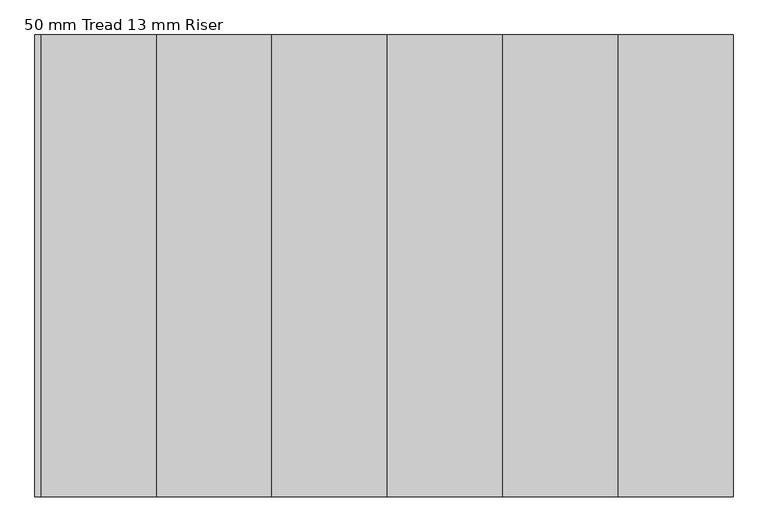
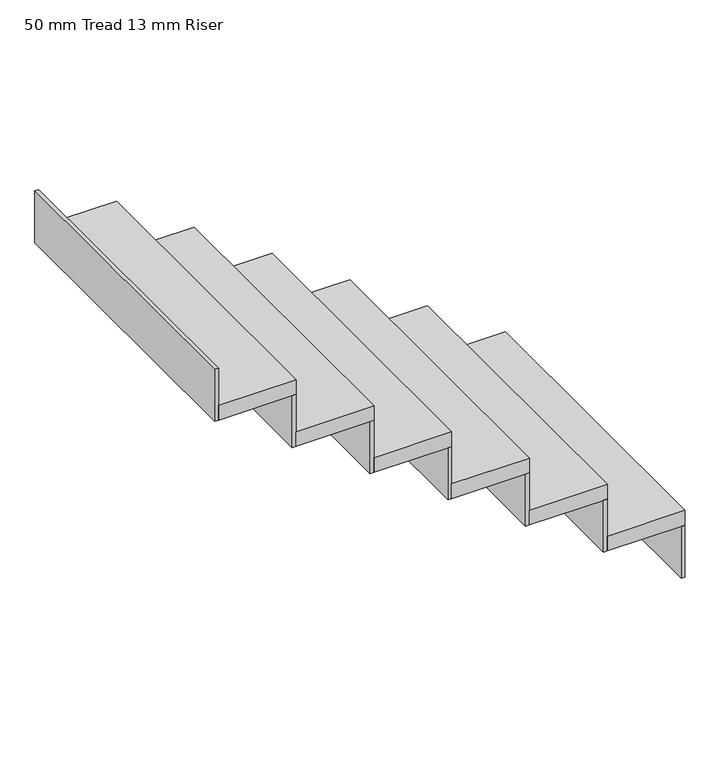
"""IFC4 building model written with IfcOpenShell, lengths in millimetres: stair flight geometry, 50 mm Tread 13 mm Riser."""

import ifcopenshell
import ifcopenshell.guid

model = None  # the IFC model being written
_history = None  # IfcOwnerHistory: only IFC2X3 demands one
_inside = {}  # id of a spatial element -> (the spatial element, [elements in it])
_under = {}  # id of a project, library or spatial element -> (it, [spatial elements below it])
_declared = {}  # id of a project -> (the project, [libraries it declares])
_typed = {}  # id of a type object -> (the type object, [elements of that type])
_made_of = {}  # id of a material, layer set ... -> (it, [elements and type objects made of it])


def new_model(schema):
    """Start an empty IFC model of exactly this schema.

    Asked for "IFC4X3", IfcOpenShell would pick the latest addendum, in which some entities
    have other attributes; the version numbers below select the first issue.
    IFC2X3 requires an IfcOwnerHistory on every rooted entity: one is made here for all.
    """
    global model, _history
    if schema == "IFC4X3":
        model = ifcopenshell.file(schema_version=(4, 3, 0, 0))
    else:
        model = ifcopenshell.file(schema=schema)
    _inside.clear()
    _under.clear()
    _declared.clear()
    _typed.clear()
    _made_of.clear()
    _history = None
    if model.schema == "IFC2X3":
        org = make("IfcOrganization", Name="unknown")
        user = make(
            "IfcPersonAndOrganization",
            ThePerson=make("IfcPerson", FamilyName="unknown"),
            TheOrganization=org,
        )
        app = make(
            "IfcApplication",
            ApplicationDeveloper=org,
            Version="unknown",
            ApplicationFullName="unknown",
            ApplicationIdentifier="unknown",
        )
        _history = make(
            "IfcOwnerHistory",
            OwningUser=user,
            OwningApplication=app,
            ChangeAction="ADDED",
            CreationDate=0,
        )
    return model


def make(cls, **values):
    """One entity of the class cls with the attributes given. An attribute that is None is left unset."""
    return model.create_entity(
        cls, **{name: value for name, value in values.items() if value is not None}
    )


def rooted(cls, **values):
    """An entity with a GlobalId (a new one), such as an element, a storey or a relation."""
    return make(cls, GlobalId=ifcopenshell.guid.new(), OwnerHistory=_history, **values)


def si_unit(unit_type, name, prefix=None):
    """IfcSIUnit, for example si_unit("LENGTHUNIT", "METRE", prefix="MILLI")."""
    return make("IfcSIUnit", UnitType=unit_type, Prefix=prefix, Name=name)


def assignment(units):
    """IfcUnitAssignment: the units of a project."""
    return None if units is None else make("IfcUnitAssignment", Units=units)


def point(xyz):
    """IfcCartesianPoint."""
    return None if xyz is None else make("IfcCartesianPoint", Coordinates=xyz)


def direction(xyz):
    """IfcDirection."""
    return None if xyz is None else make("IfcDirection", DirectionRatios=xyz)


def frame(location, z_axis=None, x_axis=None):
    """IfcAxis2Placement3D, a coordinate frame: its origin and axes. An axis left out is left unset."""
    return make(
        "IfcAxis2Placement3D",
        Location=point(location),
        Axis=direction(z_axis),
        RefDirection=direction(x_axis),
    )


def origin():
    """The frame at (0, 0, 0) with its axes left unset."""
    return frame((0.0, 0.0, 0.0))


def place(relative_to, where):
    """IfcLocalPlacement: puts the frame where relative to a parent placement (None: the world)."""
    return make(
        "IfcLocalPlacement", PlacementRelTo=relative_to, RelativePlacement=where
    )


def context(
    kind, dimensions, precision=None, world=None, true_north=None, identifier=None
):
    """IfcGeometricRepresentationContext, for example the 3D "Model" context."""
    return make(
        "IfcGeometricRepresentationContext",
        ContextIdentifier=identifier,
        ContextType=kind,
        CoordinateSpaceDimension=dimensions,
        Precision=precision,
        WorldCoordinateSystem=world,
        TrueNorth=true_north,
    )


def project(units=None, contexts=None):
    """IfcProject with its units and contexts."""
    return rooted(
        "IfcProject",
        Name="project",
        RepresentationContexts=contexts,
        UnitsInContext=assignment(units),
    )


def spatial(cls, under=None, at=None, **own):
    """A site, building, storey or space (cls), placed at a placement, below another one or the project."""
    s = rooted(cls, ObjectPlacement=at, **own)
    if under is not None:
        _under.setdefault(under.id(), (under, []))[1].append(s)
    return s


def polyline(points):
    """IfcPolyline through the points."""
    return make("IfcPolyline", Points=[point(p) for p in points])


def outline(outer, holes=None, kind="AREA"):
    """IfcArbitraryClosedProfileDef: a profile drawn as a closed curve; with holes, ...WithVoids."""
    if holes is None:
        return make("IfcArbitraryClosedProfileDef", ProfileType=kind, OuterCurve=outer)
    return make(
        "IfcArbitraryProfileDefWithVoids",
        ProfileType=kind,
        OuterCurve=outer,
        InnerCurves=holes,
    )


def extrude(swept, where, along, depth):
    """IfcExtrudedAreaSolid: the profile swept, set in the frame where, extruded along a direction by depth."""
    return make(
        "IfcExtrudedAreaSolid",
        SweptArea=swept,
        Position=where,
        ExtrudedDirection=direction(along),
        Depth=depth,
    )


def shape(context_of_items, identifier, shape_type, items):
    """IfcShapeRepresentation: the items that make up one representation, for example the "Body"."""
    return make(
        "IfcShapeRepresentation",
        ContextOfItems=context_of_items,
        RepresentationIdentifier=identifier,
        RepresentationType=shape_type,
        Items=items,
    )


def source(mapping_origin, context_of_items, identifier, shape_type, items):
    """IfcRepresentationMap: a shape defined once, which mapped items show again and again."""
    return make(
        "IfcRepresentationMap",
        MappingOrigin=mapping_origin,
        MappedRepresentation=shape(context_of_items, identifier, shape_type, items),
    )


def transform(
    local_origin,
    x_axis=None,
    y_axis=None,
    z_axis=None,
    scale=None,
    scale2=None,
    scale3=None,
    uniform=True,
):
    """IfcCartesianTransformationOperator3D, or its non-uniform kind. x_axis, y_axis, z_axis: its Axis1, 2, 3."""
    if uniform:
        return make(
            "IfcCartesianTransformationOperator3D",
            Axis1=direction(x_axis),
            Axis2=direction(y_axis),
            LocalOrigin=point(local_origin),
            Scale=scale,
            Axis3=direction(z_axis),
        )
    return make(
        "IfcCartesianTransformationOperator3DnonUniform",
        Axis1=direction(x_axis),
        Axis2=direction(y_axis),
        LocalOrigin=point(local_origin),
        Scale=scale,
        Axis3=direction(z_axis),
        Scale2=scale2,
        Scale3=scale3,
    )


def mapped(mapping_source, mapping_target):
    """IfcMappedItem: shows the shape of a source again, moved by a transform."""
    return make(
        "IfcMappedItem", MappingSource=mapping_source, MappingTarget=mapping_target
    )


def made_of(thing, what):
    """Note that an element or type object is made of a material, layer set ...; save() writes the relation."""
    if what is not None:
        _made_of.setdefault(what.id(), (what, []))[1].append(thing)
    return thing


def element(
    cls,
    number,
    at=None,
    inside=None,
    cuts=None,
    type_object=None,
    material=None,
    context=None,
    identifier="Body",
    shape_type=None,
    held_by="IfcProductDefinitionShape",
    body=None,
    shapes=None,
    **own,
):
    """One element of the class cls, such as IfcWall. Its Tag is "e" and its number.

    at: its placement. inside: the storey or other place that contains it. cuts: it is an
    opening in that element (IfcRelVoidsElement). A single representation is given by context,
    identifier, shape_type and body (its items); several are given by shapes. held_by: the class
    of the entity that holds the representations. save() writes the other relations.
    """
    e = rooted(cls, Tag="e%d" % number, ObjectPlacement=at, **own)
    if body is not None:
        shapes = [shape(context, identifier, shape_type, body)]
    if shapes is not None:
        e.Representation = make(held_by, Representations=shapes)
    if inside is not None:
        _inside.setdefault(inside.id(), (inside, []))[1].append(e)
    if cuts is not None:
        rooted(
            "IfcRelVoidsElement", RelatingBuildingElement=cuts, RelatedOpeningElement=e
        )
    if type_object is not None:
        _typed.setdefault(type_object.id(), (type_object, []))[1].append(e)
    return made_of(e, material)


def aggregate(whole, parts):
    """IfcRelAggregates: a whole, such as a stair, and the parts it consists of."""
    return rooted("IfcRelAggregates", RelatingObject=whole, RelatedObjects=parts)


def save(model, path):
    """Write the relations noted so far, then the file.

    IfcRelAggregates (storeys below a building ...), IfcRelContainedInSpatialStructure (elements
    in a storey), IfcRelDefinesByType, IfcRelAssociatesMaterial and IfcRelDeclares: one each for
    every whole, place, type object, material and project.
    """
    for whole, parts in _under.values():
        aggregate(whole, parts)
    for where, things in _inside.values():
        rooted(
            "IfcRelContainedInSpatialStructure",
            RelatedElements=things,
            RelatingStructure=where,
        )
    for kind, things in _typed.values():
        rooted("IfcRelDefinesByType", RelatedObjects=things, RelatingType=kind)
    for what, things in _made_of.values():
        rooted("IfcRelAssociatesMaterial", RelatedObjects=things, RelatingMaterial=what)
    for by, libraries in _declared.values():
        rooted("IfcRelDeclares", RelatingContext=by, RelatedDefinitions=libraries)
    model.write(path)


def stair_flight_50_mm_tread_13_mm_riser_2f4f0ea2(model_context):
    return source(origin(), model_context, "Body", "SweptSolid", [
        extrude(outline(polyline([(10138.2119026, -838.2971943), (10150.7119026, -838.2971943), (10150.7119026, -1838.2971943), (10138.2119026, -1838.2971943), (10138.2119026, -838.2971943)])), frame((0.0, 0.0, 1714.7058824), z_axis=(0.0, 0.0, 1.0), x_axis=(1.0, 0.0, 0.0)), (0.0, 0.0, 1.0), 176.4705882),
        extrude(outline(polyline([(9900.7119026, -1838.2971943), (9900.7119026, -838.2971943), (10150.7119026, -838.2971943), (10150.7119026, -1838.2971943), (9900.7119026, -1838.2971943)])), frame((0.0, 0.0, 1891.1764706), z_axis=(0.0, 0.0, 1.0), x_axis=(1.0, 0.0, 0.0)), (0.0, 0.0, 1.0), 50.0),
        extrude(outline(polyline([(9888.2119026, -838.2971943), (9900.7119026, -838.2971943), (9900.7119026, -1838.2971943), (9888.2119026, -1838.2971943), (9888.2119026, -838.2971943)])), frame((0.0, 0.0, 1891.1764706), z_axis=(0.0, 0.0, 1.0), x_axis=(1.0, 0.0, 0.0)), (0.0, 0.0, 1.0), 176.4705882),
        extrude(outline(polyline([(9650.7119026, -1838.2971943), (9650.7119026, -838.2971943), (9900.7119026, -838.2971943), (9900.7119026, -1838.2971943), (9650.7119026, -1838.2971943)])), frame((0.0, 0.0, 2067.6470588), z_axis=(0.0, 0.0, 1.0), x_axis=(1.0, 0.0, 0.0)), (0.0, 0.0, 1.0), 50.0),
        extrude(outline(polyline([(9638.2119026, -838.2971943), (9650.7119026, -838.2971943), (9650.7119026, -1838.2971943), (9638.2119026, -1838.2971943), (9638.2119026, -838.2971943)])), frame((0.0, 0.0, 2067.6470588), z_axis=(0.0, 0.0, 1.0), x_axis=(1.0, 0.0, 0.0)), (0.0, 0.0, 1.0), 176.4705882),
        extrude(outline(polyline([(9400.7119026, -1838.2971943), (9400.7119026, -838.2971943), (9650.7119026, -838.2971943), (9650.7119026, -1838.2971943), (9400.7119026, -1838.2971943)])), frame((0.0, 0.0, 2244.1176471), z_axis=(0.0, 0.0, 1.0), x_axis=(1.0, 0.0, 0.0)), (0.0, 0.0, 1.0), 50.0),
        extrude(outline(polyline([(9388.2119026, -838.2971943), (9400.7119026, -838.2971943), (9400.7119026, -1838.2971943), (9388.2119026, -1838.2971943), (9388.2119026, -838.2971943)])), frame((0.0, 0.0, 2244.1176471), z_axis=(0.0, 0.0, 1.0), x_axis=(1.0, 0.0, 0.0)), (0.0, 0.0, 1.0), 176.4705882),
        extrude(outline(polyline([(9150.7119026, -1838.2971943), (9150.7119026, -838.2971943), (9400.7119026, -838.2971943), (9400.7119026, -1838.2971943), (9150.7119026, -1838.2971943)])), frame((0.0, 0.0, 2420.5882353), z_axis=(0.0, 0.0, 1.0), x_axis=(1.0, 0.0, 0.0)), (0.0, 0.0, 1.0), 50.0),
        extrude(outline(polyline([(9138.2119026, -838.2971943), (9150.7119026, -838.2971943), (9150.7119026, -1838.2971943), (9138.2119026, -1838.2971943), (9138.2119026, -838.2971943)])), frame((0.0, 0.0, 2420.5882353), z_axis=(0.0, 0.0, 1.0), x_axis=(1.0, 0.0, 0.0)), (0.0, 0.0, 1.0), 176.4705882),
        extrude(outline(polyline([(8900.7119026, -1838.2971943), (8900.7119026, -838.2971943), (9150.7119026, -838.2971943), (9150.7119026, -1838.2971943), (8900.7119026, -1838.2971943)])), frame((0.0, 0.0, 2597.0588235), z_axis=(0.0, 0.0, 1.0), x_axis=(1.0, 0.0, 0.0)), (0.0, 0.0, 1.0), 50.0),
        extrude(outline(polyline([(8888.2119026, -838.2971943), (8900.7119026, -838.2971943), (8900.7119026, -1838.2971943), (8888.2119026, -1838.2971943), (8888.2119026, -838.2971943)])), frame((0.0, 0.0, 2597.0588235), z_axis=(0.0, 0.0, 1.0), x_axis=(1.0, 0.0, 0.0)), (0.0, 0.0, 1.0), 176.4705882),
        extrude(outline(polyline([(8638.2119026, -838.2971943), (8650.7119026, -838.2971943), (8650.7119026, -1838.2971943), (8638.2119026, -1838.2971943), (8638.2119026, -838.2971943)])), frame((0.0, 0.0, 2773.5294118), z_axis=(0.0, 0.0, 1.0), x_axis=(1.0, 0.0, 0.0)), (0.0, 0.0, 1.0), 176.4705882),
        extrude(outline(polyline([(8650.7119026, -1838.2971943), (8650.7119026, -838.2971943), (8900.7119026, -838.2971943), (8900.7119026, -1838.2971943), (8650.7119026, -1838.2971943)])), frame((0.0, 0.0, 2773.5294118), z_axis=(0.0, 0.0, 1.0), x_axis=(1.0, 0.0, 0.0)), (0.0, 0.0, 1.0), 50.0),
    ])


if __name__ == "__main__":
    model = new_model("IFC4")
    model_context = context("Model", 3, world=origin())
    ifc_project = project(units=[si_unit("LENGTHUNIT", "METRE", prefix="MILLI")], contexts=[model_context])
    site = spatial("IfcSite", under=ifc_project)
    building = spatial("IfcBuilding", under=site)
    placement = place(None, origin())
    stair_flight_50_mm_tread_13_mm_riser_shape = stair_flight_50_mm_tread_13_mm_riser_2f4f0ea2(model_context)
    element("IfcStairFlight", 1, ObjectType="50 mm Tread 13 mm Riser", at=placement, inside=building, context=model_context, shape_type="MappedRepresentation", body=[
        mapped(stair_flight_50_mm_tread_13_mm_riser_shape, transform((0.0, 0.0, 0.0), x_axis=(1.0, 0.0, 0.0), y_axis=(0.0, 1.0, 0.0), z_axis=(0.0, 0.0, 1.0))),
    ])
    save(model, "model.ifc")
